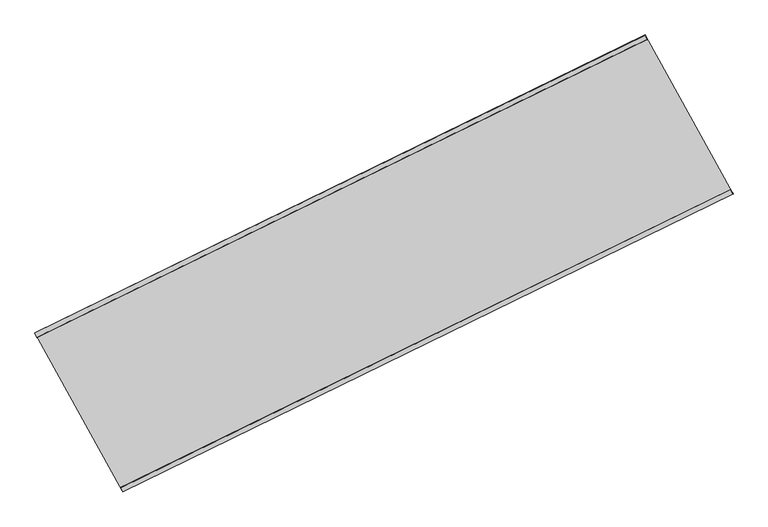
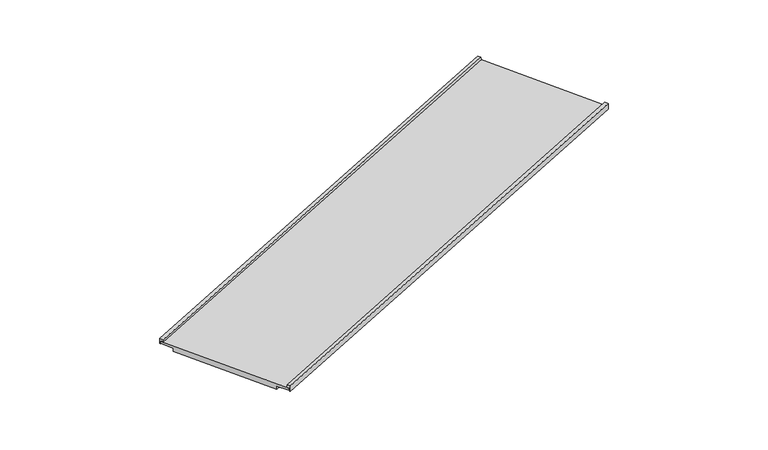
"""IFC4 building model written with IfcOpenShell, lengths in millimetres: beam geometry, KNA_SF_Brugdek : Brugdek."""

from ifc_helpers import new_model, si_unit, frame, origin, place, context, project, spatial, polyline, outline, extrude, faceted_brep, source, transform, mapped, element, save


def beam_f54b55c9(model_context):
    return source(origin(), model_context, "Body", "SolidModel", [
        extrude(outline(polyline([(19.9925463, -20.0), (19.9925463, 310.0), (300.0, 280.0), (300.0000001, -120.0000001), (-350.0, -120.0), (-350.0, -20.0000001), (19.9925463, -20.0)])), frame((114201.377241, -43988.5484331, 4665.5216838), z_axis=(0.8981217866158243, 0.4390028664450355, 0.025568333129915705), x_axis=(-0.01200466238246137, -0.033645258728366455, 0.9993617386343068)), (0.0, 0.0, 1.0), 58694.8205232),
        extrude(outline(polyline([(20.0, -20.0000001), (20.0, 349.9999999), (120.0, 349.9999999), (120.0000001, -350.0), (-280.0, -350.0), (-315.3571428, -20.0000001), (20.0, -20.0000001)])), frame((121687.6762788, -57511.1982285, 4300.1859455), z_axis=(0.8981217866158244, 0.43900286644503533, 0.025568333129915723), x_axis=(0.4391464336326592, -0.8984154995477964, 0.0)), (0.0, 0.0, 1.0), 58694.8205232),
        faceted_brep([(167643.9332384, -19535.3773986, 5430.3029219), (114928.836165, -45302.5718537, 3929.5741978), (114928.836165, -45302.5718537, 4317.364139), (167643.9332384, -19535.3773986, 5818.0928631), (114201.377241, -43988.5484331, 4415.4399263), (166916.4743144, -18221.3539779, 5916.1686504), (114201.377241, -43988.5484331, 4665.5216838), (166916.4743144, -18221.3539779, 6166.250408), (121687.6762788, -57511.1982285, 4300.1859455), (174402.7733522, -31744.0037733, 5800.9146697), (121687.6762788, -57511.1982285, 4049.9742507), (174402.7733522, -31744.0037733, 5550.7029748), (120960.2173548, -56197.1748078, 4023.0292361), (173675.3144282, -30429.9803527, 5523.7579603), (120960.2173548, -56197.1748078, 3635.2392949), (173675.3144282, -30429.9803527, 5135.9680191)], [[[0, 1, 2, 3]], [[3, 2, 4, 5]], [[5, 4, 6, 7]], [[7, 6, 8, 9]], [[9, 8, 10, 11]], [[11, 10, 12, 13]], [[13, 12, 14, 15]], [[1, 0, 15, 14]], [[0, 3, 5, 7, 9, 11, 13, 15]], [[2, 1, 14, 12, 10, 8, 6, 4]]]),
    ])


if __name__ == "__main__":
    model = new_model("IFC4")
    model_context = context("Model", 3, world=origin())
    ifc_project = project(units=[si_unit("LENGTHUNIT", "METRE", prefix="MILLI")], contexts=[model_context])
    site = spatial("IfcSite", under=ifc_project)
    building = spatial("IfcBuilding", under=site)
    placement = place(None, origin())
    beam_shape = beam_f54b55c9(model_context)
    element("IfcBeam", 1, ObjectType="KNA_SF_Brugdek : Brugdek", at=placement, inside=building, context=model_context, shape_type="MappedRepresentation", body=[
        mapped(beam_shape, transform((0.0, 0.0, 0.0), x_axis=(1.0, 0.0, 0.0), y_axis=(0.0, 1.0, 0.0), z_axis=(0.0, 0.0, 1.0))),
    ])
    save(model, "model.ifc")
